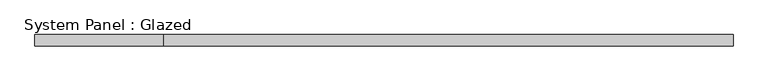
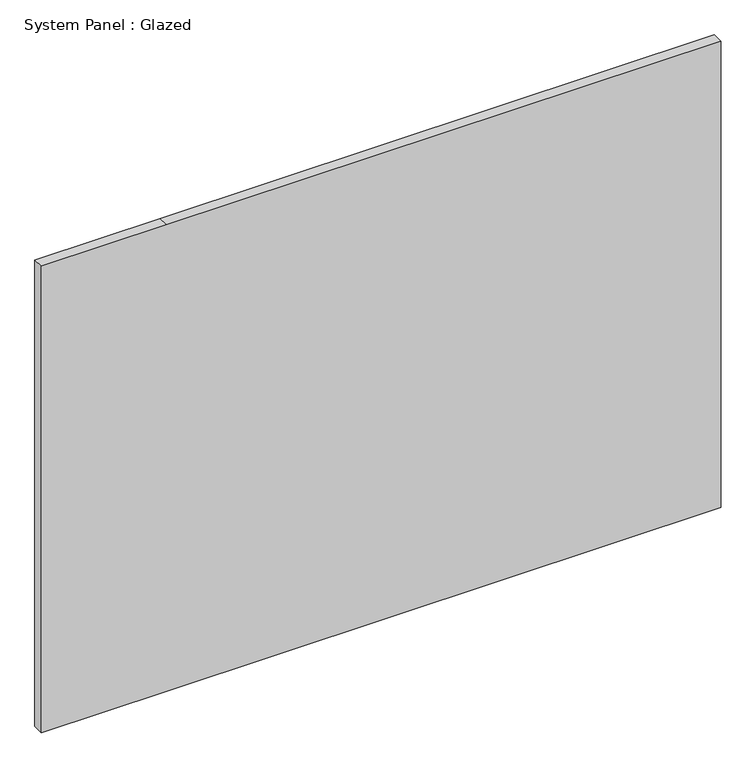
"""IFC4 building model written with IfcOpenShell, lengths in millimetres: plate geometry, System Panel : Glazed."""

from ifc_helpers import new_model, si_unit, frame, origin, place, context, project, spatial, polyline, outline, extrude, source, transform, mapped, element, save


def system_panel_glazed_835a6d4f(model_context):
    return source(origin(), model_context, "Body", "SweptSolid", [
        extrude(outline(polyline([(0.0, -774.7), (0.0, -488.95), (0.0, 774.7), (1123.95, 774.7), (1123.95, -488.95), (1123.95, -774.7), (0.0, -774.7)])), frame((0.0, 19.05, 0.0), z_axis=(0.0, 1.0, 0.0), x_axis=(0.0, 0.0, 1.0)), (0.0, 0.0, 1.0), 25.4),
    ])


if __name__ == "__main__":
    model = new_model("IFC4")
    model_context = context("Model", 3, world=origin())
    ifc_project = project(units=[si_unit("LENGTHUNIT", "METRE", prefix="MILLI")], contexts=[model_context])
    site = spatial("IfcSite", under=ifc_project)
    building = spatial("IfcBuilding", under=site)
    placement = place(None, origin())
    system_panel_glazed_shape = system_panel_glazed_835a6d4f(model_context)
    element("IfcPlate", 1, ObjectType="System Panel : Glazed", at=placement, inside=building, context=model_context, shape_type="MappedRepresentation", body=[
        mapped(system_panel_glazed_shape, transform((0.0, 0.0, 0.0), x_axis=(1.0, 0.0, 0.0), y_axis=(0.0, 1.0, 0.0), z_axis=(0.0, 0.0, 1.0))),
    ])
    save(model, "model.ifc")

# Revit data of these elements
# Element 1 (IfcPlate, "System Panel : Glazed")
#   Materials on its faces: "Glass"
# Materials
#   "Glass": class "Glass", colour RGB 0 128 192, transparency 0.75, Cost = 0
